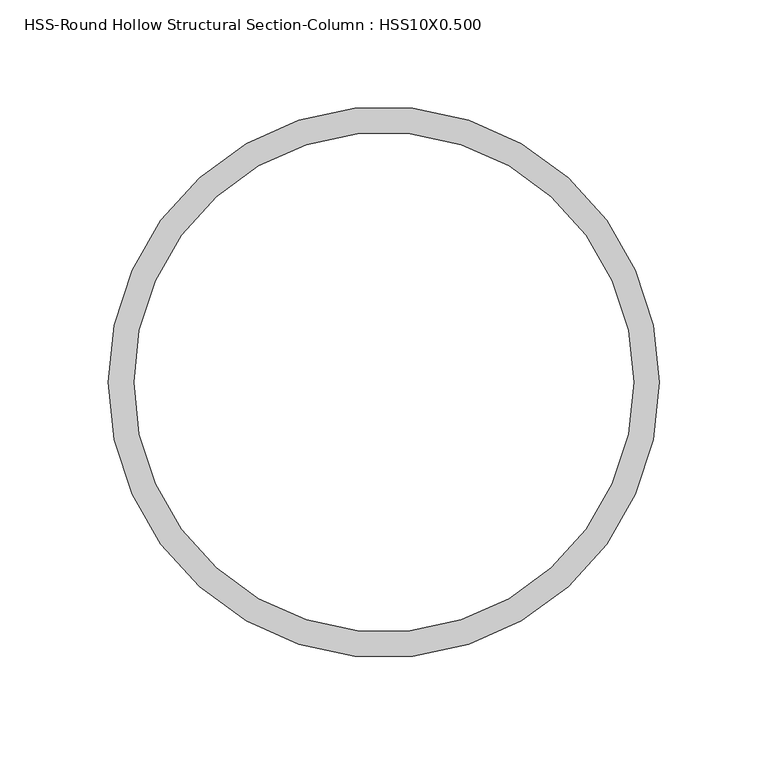
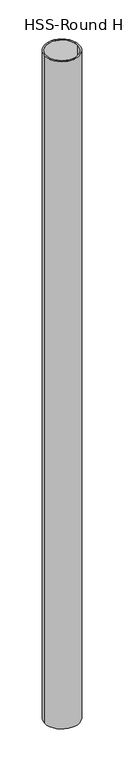
"""IFC4 building model written with IfcOpenShell, lengths in millimetres: column geometry, HSS-Round Hollow Structural Section-Column : HSS10X0.500."""

import ifcopenshell
import ifcopenshell.guid

model = None  # the IFC model being written
_history = None  # IfcOwnerHistory: only IFC2X3 demands one
_inside = {}  # id of a spatial element -> (the spatial element, [elements in it])
_under = {}  # id of a project, library or spatial element -> (it, [spatial elements below it])
_declared = {}  # id of a project -> (the project, [libraries it declares])
_typed = {}  # id of a type object -> (the type object, [elements of that type])
_made_of = {}  # id of a material, layer set ... -> (it, [elements and type objects made of it])


def new_model(schema):
    """Start an empty IFC model of exactly this schema.

    Asked for "IFC4X3", IfcOpenShell would pick the latest addendum, in which some entities
    have other attributes; the version numbers below select the first issue.
    IFC2X3 requires an IfcOwnerHistory on every rooted entity: one is made here for all.
    """
    global model, _history
    if schema == "IFC4X3":
        model = ifcopenshell.file(schema_version=(4, 3, 0, 0))
    else:
        model = ifcopenshell.file(schema=schema)
    _inside.clear()
    _under.clear()
    _declared.clear()
    _typed.clear()
    _made_of.clear()
    _history = None
    if model.schema == "IFC2X3":
        org = make("IfcOrganization", Name="unknown")
        user = make(
            "IfcPersonAndOrganization",
            ThePerson=make("IfcPerson", FamilyName="unknown"),
            TheOrganization=org,
        )
        app = make(
            "IfcApplication",
            ApplicationDeveloper=org,
            Version="unknown",
            ApplicationFullName="unknown",
            ApplicationIdentifier="unknown",
        )
        _history = make(
            "IfcOwnerHistory",
            OwningUser=user,
            OwningApplication=app,
            ChangeAction="ADDED",
            CreationDate=0,
        )
    return model


def make(cls, **values):
    """One entity of the class cls with the attributes given. An attribute that is None is left unset."""
    return model.create_entity(
        cls, **{name: value for name, value in values.items() if value is not None}
    )


def rooted(cls, **values):
    """An entity with a GlobalId (a new one), such as an element, a storey or a relation."""
    return make(cls, GlobalId=ifcopenshell.guid.new(), OwnerHistory=_history, **values)


def si_unit(unit_type, name, prefix=None):
    """IfcSIUnit, for example si_unit("LENGTHUNIT", "METRE", prefix="MILLI")."""
    return make("IfcSIUnit", UnitType=unit_type, Prefix=prefix, Name=name)


def assignment(units):
    """IfcUnitAssignment: the units of a project."""
    return None if units is None else make("IfcUnitAssignment", Units=units)


def point(xyz):
    """IfcCartesianPoint."""
    return None if xyz is None else make("IfcCartesianPoint", Coordinates=xyz)


def direction(xyz):
    """IfcDirection."""
    return None if xyz is None else make("IfcDirection", DirectionRatios=xyz)


def frame(location, z_axis=None, x_axis=None):
    """IfcAxis2Placement3D, a coordinate frame: its origin and axes. An axis left out is left unset."""
    return make(
        "IfcAxis2Placement3D",
        Location=point(location),
        Axis=direction(z_axis),
        RefDirection=direction(x_axis),
    )


def frame_2d(location, x_axis=None):
    """IfcAxis2Placement2D, a coordinate frame in the plane: its origin and x axis."""
    return make(
        "IfcAxis2Placement2D", Location=point(location), RefDirection=direction(x_axis)
    )


def origin():
    """The frame at (0, 0, 0) with its axes left unset."""
    return frame((0.0, 0.0, 0.0))


def origin_2d():
    """The frame at (0, 0) in the plane with its x axis left unset."""
    return frame_2d((0.0, 0.0))


def place(relative_to, where):
    """IfcLocalPlacement: puts the frame where relative to a parent placement (None: the world)."""
    return make(
        "IfcLocalPlacement", PlacementRelTo=relative_to, RelativePlacement=where
    )


def context(
    kind, dimensions, precision=None, world=None, true_north=None, identifier=None
):
    """IfcGeometricRepresentationContext, for example the 3D "Model" context."""
    return make(
        "IfcGeometricRepresentationContext",
        ContextIdentifier=identifier,
        ContextType=kind,
        CoordinateSpaceDimension=dimensions,
        Precision=precision,
        WorldCoordinateSystem=world,
        TrueNorth=true_north,
    )


def project(units=None, contexts=None):
    """IfcProject with its units and contexts."""
    return rooted(
        "IfcProject",
        Name="project",
        RepresentationContexts=contexts,
        UnitsInContext=assignment(units),
    )


def spatial(cls, under=None, at=None, **own):
    """A site, building, storey or space (cls), placed at a placement, below another one or the project."""
    s = rooted(cls, ObjectPlacement=at, **own)
    if under is not None:
        _under.setdefault(under.id(), (under, []))[1].append(s)
    return s


def circle_curve(where, radius):
    """IfcCircle in the frame where."""
    return make("IfcCircle", Position=where, Radius=radius)


def trimmed(basis, trim1, trim2, sense, master):
    """IfcTrimmedCurve: the piece of a basis curve between two trims."""
    return make(
        "IfcTrimmedCurve",
        BasisCurve=basis,
        Trim1=trim1,
        Trim2=trim2,
        SenseAgreement=sense,
        MasterRepresentation=master,
    )


def segment(curve, same_sense, transition):
    """IfcCompositeCurveSegment."""
    return make(
        "IfcCompositeCurveSegment",
        Transition=transition,
        SameSense=same_sense,
        ParentCurve=curve,
    )


def composite_curve(segments, self_intersect=None):
    """IfcCompositeCurve: segments joined end to end."""
    return make("IfcCompositeCurve", Segments=segments, SelfIntersect=self_intersect)


def outline(outer, holes=None, kind="AREA"):
    """IfcArbitraryClosedProfileDef: a profile drawn as a closed curve; with holes, ...WithVoids."""
    if holes is None:
        return make("IfcArbitraryClosedProfileDef", ProfileType=kind, OuterCurve=outer)
    return make(
        "IfcArbitraryProfileDefWithVoids",
        ProfileType=kind,
        OuterCurve=outer,
        InnerCurves=holes,
    )


def extrude(swept, where, along, depth):
    """IfcExtrudedAreaSolid: the profile swept, set in the frame where, extruded along a direction by depth."""
    return make(
        "IfcExtrudedAreaSolid",
        SweptArea=swept,
        Position=where,
        ExtrudedDirection=direction(along),
        Depth=depth,
    )


def shape(context_of_items, identifier, shape_type, items):
    """IfcShapeRepresentation: the items that make up one representation, for example the "Body"."""
    return make(
        "IfcShapeRepresentation",
        ContextOfItems=context_of_items,
        RepresentationIdentifier=identifier,
        RepresentationType=shape_type,
        Items=items,
    )


def source(mapping_origin, context_of_items, identifier, shape_type, items):
    """IfcRepresentationMap: a shape defined once, which mapped items show again and again."""
    return make(
        "IfcRepresentationMap",
        MappingOrigin=mapping_origin,
        MappedRepresentation=shape(context_of_items, identifier, shape_type, items),
    )


def transform(
    local_origin,
    x_axis=None,
    y_axis=None,
    z_axis=None,
    scale=None,
    scale2=None,
    scale3=None,
    uniform=True,
):
    """IfcCartesianTransformationOperator3D, or its non-uniform kind. x_axis, y_axis, z_axis: its Axis1, 2, 3."""
    if uniform:
        return make(
            "IfcCartesianTransformationOperator3D",
            Axis1=direction(x_axis),
            Axis2=direction(y_axis),
            LocalOrigin=point(local_origin),
            Scale=scale,
            Axis3=direction(z_axis),
        )
    return make(
        "IfcCartesianTransformationOperator3DnonUniform",
        Axis1=direction(x_axis),
        Axis2=direction(y_axis),
        LocalOrigin=point(local_origin),
        Scale=scale,
        Axis3=direction(z_axis),
        Scale2=scale2,
        Scale3=scale3,
    )


def mapped(mapping_source, mapping_target):
    """IfcMappedItem: shows the shape of a source again, moved by a transform."""
    return make(
        "IfcMappedItem", MappingSource=mapping_source, MappingTarget=mapping_target
    )


def made_of(thing, what):
    """Note that an element or type object is made of a material, layer set ...; save() writes the relation."""
    if what is not None:
        _made_of.setdefault(what.id(), (what, []))[1].append(thing)
    return thing


def element(
    cls,
    number,
    at=None,
    inside=None,
    cuts=None,
    type_object=None,
    material=None,
    context=None,
    identifier="Body",
    shape_type=None,
    held_by="IfcProductDefinitionShape",
    body=None,
    shapes=None,
    **own,
):
    """One element of the class cls, such as IfcWall. Its Tag is "e" and its number.

    at: its placement. inside: the storey or other place that contains it. cuts: it is an
    opening in that element (IfcRelVoidsElement). A single representation is given by context,
    identifier, shape_type and body (its items); several are given by shapes. held_by: the class
    of the entity that holds the representations. save() writes the other relations.
    """
    e = rooted(cls, Tag="e%d" % number, ObjectPlacement=at, **own)
    if body is not None:
        shapes = [shape(context, identifier, shape_type, body)]
    if shapes is not None:
        e.Representation = make(held_by, Representations=shapes)
    if inside is not None:
        _inside.setdefault(inside.id(), (inside, []))[1].append(e)
    if cuts is not None:
        rooted(
            "IfcRelVoidsElement", RelatingBuildingElement=cuts, RelatedOpeningElement=e
        )
    if type_object is not None:
        _typed.setdefault(type_object.id(), (type_object, []))[1].append(e)
    return made_of(e, material)


def aggregate(whole, parts):
    """IfcRelAggregates: a whole, such as a stair, and the parts it consists of."""
    return rooted("IfcRelAggregates", RelatingObject=whole, RelatedObjects=parts)


def save(model, path):
    """Write the relations noted so far, then the file.

    IfcRelAggregates (storeys below a building ...), IfcRelContainedInSpatialStructure (elements
    in a storey), IfcRelDefinesByType, IfcRelAssociatesMaterial and IfcRelDeclares: one each for
    every whole, place, type object, material and project.
    """
    for whole, parts in _under.values():
        aggregate(whole, parts)
    for where, things in _inside.values():
        rooted(
            "IfcRelContainedInSpatialStructure",
            RelatedElements=things,
            RelatingStructure=where,
        )
    for kind, things in _typed.values():
        rooted("IfcRelDefinesByType", RelatedObjects=things, RelatingType=kind)
    for what, things in _made_of.values():
        rooted("IfcRelAssociatesMaterial", RelatedObjects=things, RelatingMaterial=what)
    for by, libraries in _declared.values():
        rooted("IfcRelDeclares", RelatingContext=by, RelatedDefinitions=libraries)
    model.write(path)


def hss_round_hollow_structural_section_column_hss10x0_500_13b5c828(model_context):
    return source(origin(), model_context, "Body", "SweptSolid", [
        extrude(outline(composite_curve([segment(trimmed(circle_curve(origin_2d(), 127.0), [point((-127.0, 0.0))], [point((127.0, 0.0))], False, "CARTESIAN"), True, "CONTINUOUS"), segment(trimmed(circle_curve(origin_2d(), 127.0), [point((127.0, 0.0))], [point((-127.0, 0.0))], False, "CARTESIAN"), True, "CONTINUOUS")], self_intersect=False), holes=[composite_curve([segment(trimmed(circle_curve(origin_2d(), 115.189), [point((-115.189, 0.0))], [point((115.189, 0.0))], True, "CARTESIAN"), True, "CONTINUOUS"), segment(trimmed(circle_curve(origin_2d(), 115.189), [point((115.189, 0.0))], [point((-115.189, 0.0))], True, "CARTESIAN"), True, "CONTINUOUS")], self_intersect=False)]), frame((0.0, 0.0, 15113.0), z_axis=(0.0, 0.0, 1.0), x_axis=(1.0, 0.0, 0.0)), (0.0, 0.0, 1.0), 5232.4),
    ])


if __name__ == "__main__":
    model = new_model("IFC4")
    model_context = context("Model", 3, world=origin())
    ifc_project = project(units=[si_unit("LENGTHUNIT", "METRE", prefix="MILLI")], contexts=[model_context])
    site = spatial("IfcSite", under=ifc_project)
    building = spatial("IfcBuilding", under=site)
    placement = place(None, origin())
    hss_round_hollow_structural_section_column_hss10x0_500_shape = hss_round_hollow_structural_section_column_hss10x0_500_13b5c828(model_context)
    element("IfcColumn", 1, ObjectType="HSS-Round Hollow Structural Section-Column : HSS10X0.500", at=placement, inside=building, context=model_context, shape_type="MappedRepresentation", body=[
        mapped(hss_round_hollow_structural_section_column_hss10x0_500_shape, transform((0.0, 0.0, 0.0), x_axis=(1.0, 0.0, 0.0), y_axis=(0.0, 1.0, 0.0), z_axis=(0.0, 0.0, 1.0))),
    ])
    save(model, "model.ifc")

# Revit data of these elements
# Type "HSS-Round Hollow Structural Section-Column : HSS10X0.500"
#   Assembly Code = "B10"
#   W = 50.8
#   OD = 0' - 10"
#   t = 0' - 0.465"
#   A = 0.0965278 SF
#   Column Material [instance default] = Metal - Steel - ASTM A53
# Element 1 (IfcColumn, "HSS-Round Hollow Structural Section-Column : HSS10X0.500")
#   Materials on its faces: "Metal - Steel - ASTM A53"
# Materials
#   "Metal - Steel - ASTM A53": class "Metal", colour RGB 128 0 0, transparency 0
